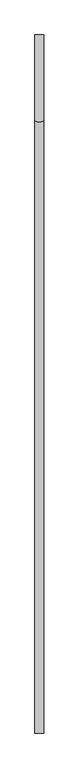
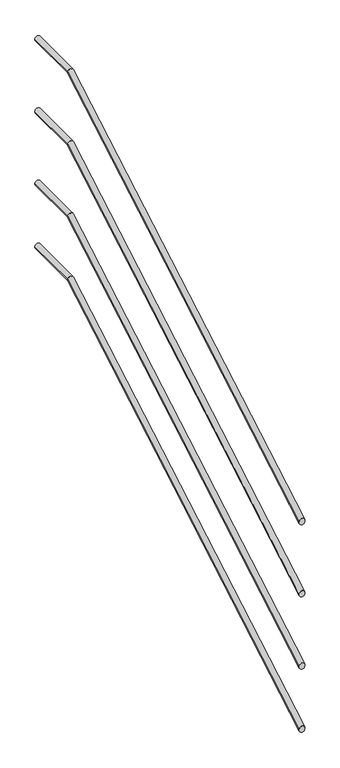
"""IFC4 building model written with IfcOpenShell, lengths in millimetres: railing geometry."""

import ifcopenshell
import ifcopenshell.guid

model = None  # the IFC model being written
_history = None  # IfcOwnerHistory: only IFC2X3 demands one
_inside = {}  # id of a spatial element -> (the spatial element, [elements in it])
_under = {}  # id of a project, library or spatial element -> (it, [spatial elements below it])
_declared = {}  # id of a project -> (the project, [libraries it declares])
_typed = {}  # id of a type object -> (the type object, [elements of that type])
_made_of = {}  # id of a material, layer set ... -> (it, [elements and type objects made of it])


def new_model(schema):
    """Start an empty IFC model of exactly this schema.

    Asked for "IFC4X3", IfcOpenShell would pick the latest addendum, in which some entities
    have other attributes; the version numbers below select the first issue.
    IFC2X3 requires an IfcOwnerHistory on every rooted entity: one is made here for all.
    """
    global model, _history
    if schema == "IFC4X3":
        model = ifcopenshell.file(schema_version=(4, 3, 0, 0))
    else:
        model = ifcopenshell.file(schema=schema)
    _inside.clear()
    _under.clear()
    _declared.clear()
    _typed.clear()
    _made_of.clear()
    _history = None
    if model.schema == "IFC2X3":
        org = make("IfcOrganization", Name="unknown")
        user = make(
            "IfcPersonAndOrganization",
            ThePerson=make("IfcPerson", FamilyName="unknown"),
            TheOrganization=org,
        )
        app = make(
            "IfcApplication",
            ApplicationDeveloper=org,
            Version="unknown",
            ApplicationFullName="unknown",
            ApplicationIdentifier="unknown",
        )
        _history = make(
            "IfcOwnerHistory",
            OwningUser=user,
            OwningApplication=app,
            ChangeAction="ADDED",
            CreationDate=0,
        )
    return model


def make(cls, **values):
    """One entity of the class cls with the attributes given. An attribute that is None is left unset."""
    return model.create_entity(
        cls, **{name: value for name, value in values.items() if value is not None}
    )


def rooted(cls, **values):
    """An entity with a GlobalId (a new one), such as an element, a storey or a relation."""
    return make(cls, GlobalId=ifcopenshell.guid.new(), OwnerHistory=_history, **values)


def si_unit(unit_type, name, prefix=None):
    """IfcSIUnit, for example si_unit("LENGTHUNIT", "METRE", prefix="MILLI")."""
    return make("IfcSIUnit", UnitType=unit_type, Prefix=prefix, Name=name)


def assignment(units):
    """IfcUnitAssignment: the units of a project."""
    return None if units is None else make("IfcUnitAssignment", Units=units)


def point(xyz):
    """IfcCartesianPoint."""
    return None if xyz is None else make("IfcCartesianPoint", Coordinates=xyz)


def direction(xyz):
    """IfcDirection."""
    return None if xyz is None else make("IfcDirection", DirectionRatios=xyz)


def frame(location, z_axis=None, x_axis=None):
    """IfcAxis2Placement3D, a coordinate frame: its origin and axes. An axis left out is left unset."""
    return make(
        "IfcAxis2Placement3D",
        Location=point(location),
        Axis=direction(z_axis),
        RefDirection=direction(x_axis),
    )


def origin():
    """The frame at (0, 0, 0) with its axes left unset."""
    return frame((0.0, 0.0, 0.0))


def place(relative_to, where):
    """IfcLocalPlacement: puts the frame where relative to a parent placement (None: the world)."""
    return make(
        "IfcLocalPlacement", PlacementRelTo=relative_to, RelativePlacement=where
    )


def context(
    kind, dimensions, precision=None, world=None, true_north=None, identifier=None
):
    """IfcGeometricRepresentationContext, for example the 3D "Model" context."""
    return make(
        "IfcGeometricRepresentationContext",
        ContextIdentifier=identifier,
        ContextType=kind,
        CoordinateSpaceDimension=dimensions,
        Precision=precision,
        WorldCoordinateSystem=world,
        TrueNorth=true_north,
    )


def project(units=None, contexts=None):
    """IfcProject with its units and contexts."""
    return rooted(
        "IfcProject",
        Name="project",
        RepresentationContexts=contexts,
        UnitsInContext=assignment(units),
    )


def spatial(cls, under=None, at=None, **own):
    """A site, building, storey or space (cls), placed at a placement, below another one or the project."""
    s = rooted(cls, ObjectPlacement=at, **own)
    if under is not None:
        _under.setdefault(under.id(), (under, []))[1].append(s)
    return s


def circle_curve(where, radius):
    """IfcCircle in the frame where."""
    return make("IfcCircle", Position=where, Radius=radius)


def ellipse_curve(where, semi_axis1, semi_axis2):
    """IfcEllipse in the frame where."""
    return make(
        "IfcEllipse", Position=where, SemiAxis1=semi_axis1, SemiAxis2=semi_axis2
    )


def shape(context_of_items, identifier, shape_type, items):
    """IfcShapeRepresentation: the items that make up one representation, for example the "Body"."""
    return make(
        "IfcShapeRepresentation",
        ContextOfItems=context_of_items,
        RepresentationIdentifier=identifier,
        RepresentationType=shape_type,
        Items=items,
    )


def source(mapping_origin, context_of_items, identifier, shape_type, items):
    """IfcRepresentationMap: a shape defined once, which mapped items show again and again."""
    return make(
        "IfcRepresentationMap",
        MappingOrigin=mapping_origin,
        MappedRepresentation=shape(context_of_items, identifier, shape_type, items),
    )


def transform(
    local_origin,
    x_axis=None,
    y_axis=None,
    z_axis=None,
    scale=None,
    scale2=None,
    scale3=None,
    uniform=True,
):
    """IfcCartesianTransformationOperator3D, or its non-uniform kind. x_axis, y_axis, z_axis: its Axis1, 2, 3."""
    if uniform:
        return make(
            "IfcCartesianTransformationOperator3D",
            Axis1=direction(x_axis),
            Axis2=direction(y_axis),
            LocalOrigin=point(local_origin),
            Scale=scale,
            Axis3=direction(z_axis),
        )
    return make(
        "IfcCartesianTransformationOperator3DnonUniform",
        Axis1=direction(x_axis),
        Axis2=direction(y_axis),
        LocalOrigin=point(local_origin),
        Scale=scale,
        Axis3=direction(z_axis),
        Scale2=scale2,
        Scale3=scale3,
    )


def mapped(mapping_source, mapping_target):
    """IfcMappedItem: shows the shape of a source again, moved by a transform."""
    return make(
        "IfcMappedItem", MappingSource=mapping_source, MappingTarget=mapping_target
    )


def made_of(thing, what):
    """Note that an element or type object is made of a material, layer set ...; save() writes the relation."""
    if what is not None:
        _made_of.setdefault(what.id(), (what, []))[1].append(thing)
    return thing


def element(
    cls,
    number,
    at=None,
    inside=None,
    cuts=None,
    type_object=None,
    material=None,
    context=None,
    identifier="Body",
    shape_type=None,
    held_by="IfcProductDefinitionShape",
    body=None,
    shapes=None,
    **own,
):
    """One element of the class cls, such as IfcWall. Its Tag is "e" and its number.

    at: its placement. inside: the storey or other place that contains it. cuts: it is an
    opening in that element (IfcRelVoidsElement). A single representation is given by context,
    identifier, shape_type and body (its items); several are given by shapes. held_by: the class
    of the entity that holds the representations. save() writes the other relations.
    """
    e = rooted(cls, Tag="e%d" % number, ObjectPlacement=at, **own)
    if body is not None:
        shapes = [shape(context, identifier, shape_type, body)]
    if shapes is not None:
        e.Representation = make(held_by, Representations=shapes)
    if inside is not None:
        _inside.setdefault(inside.id(), (inside, []))[1].append(e)
    if cuts is not None:
        rooted(
            "IfcRelVoidsElement", RelatingBuildingElement=cuts, RelatedOpeningElement=e
        )
    if type_object is not None:
        _typed.setdefault(type_object.id(), (type_object, []))[1].append(e)
    return made_of(e, material)


def aggregate(whole, parts):
    """IfcRelAggregates: a whole, such as a stair, and the parts it consists of."""
    return rooted("IfcRelAggregates", RelatingObject=whole, RelatedObjects=parts)


def save(model, path):
    """Write the relations noted so far, then the file.

    IfcRelAggregates (storeys below a building ...), IfcRelContainedInSpatialStructure (elements
    in a storey), IfcRelDefinesByType, IfcRelAssociatesMaterial and IfcRelDeclares: one each for
    every whole, place, type object, material and project.
    """
    for whole, parts in _under.values():
        aggregate(whole, parts)
    for where, things in _inside.values():
        rooted(
            "IfcRelContainedInSpatialStructure",
            RelatedElements=things,
            RelatingStructure=where,
        )
    for kind, things in _typed.values():
        rooted("IfcRelDefinesByType", RelatedObjects=things, RelatingType=kind)
    for what, things in _made_of.values():
        rooted("IfcRelAssociatesMaterial", RelatedObjects=things, RelatingMaterial=what)
    for by, libraries in _declared.values():
        rooted("IfcRelDeclares", RelatingContext=by, RelatedDefinitions=libraries)
    model.write(path)


def plane_surface(at):
    """IfcPlane: the flat surface through the origin of the frame at, square to its z axis."""
    return make("IfcPlane", Position=at)


def cylinder_surface(at, radius):
    """IfcCylindricalSurface: all points at the distance radius from the z axis of the frame at."""
    return make("IfcCylindricalSurface", Position=at, Radius=radius)


def advanced_brep(points, edges, surfaces, faces):
    """IfcAdvancedBrep: a solid bounded by faces that lie on surfaces and meet in shared edges.

    An edge is (start, end): straight between two places in points (the first is 0);
    or (start, end, curve); or (start, end, curve, False) where it runs against its curve.
    A face is (place in surfaces, loops), or (place, loops, False) where it looks against
    its surface's normal. A loop lists edges by number (the first is 1), with a minus sign
    where the edge is run from its end to its start. The first loop is the outer one.
    """
    corners = [point(p) for p in points]
    vertices = [make("IfcVertexPoint", VertexGeometry=c) for c in corners]
    made = []
    for start, end, *more in edges:
        made.append(
            make(
                "IfcEdgeCurve",
                EdgeStart=vertices[start],
                EdgeEnd=vertices[end],
                EdgeGeometry=more[0] if more else make("IfcPolyline", Points=[corners[start], corners[end]]),
                SameSense=more[1] if len(more) > 1 else True,
            )
        )
    hull = []
    for where, loops, *sense in faces:
        bounds = []
        for j, loop in enumerate(loops):
            ring = [make("IfcOrientedEdge", EdgeElement=made[abs(k) - 1], Orientation=k > 0) for k in loop]
            bounds.append(
                make(
                    "IfcFaceOuterBound" if j == 0 else "IfcFaceBound",
                    Bound=make("IfcEdgeLoop", EdgeList=ring),
                    Orientation=True,
                )
            )
        hull.append(make("IfcAdvancedFace", Bounds=bounds, FaceSurface=surfaces[where], SameSense=sense[0] if sense else True))
    return make("IfcAdvancedBrep", Outer=make("IfcClosedShell", CfsFaces=hull))


def railing_e49ed630(model_context):
    return source(origin(), model_context, "Body", "AdvancedBrep", [
        advanced_brep(
        [(-1890.4, 13399.5208589, 1336.7361432), (-1860.4, 13399.5208589, 1336.7361432), (-1890.4, 15503.5584173, 2557.9030398), (-1860.4, 15503.5584173, 2557.9030398), (-1890.4, 15799.5208589, 2557.9030398), (-1860.4, 15799.5208589, 2557.9030398)],
        [
            (0, 1, ellipse_curve(frame((-1875.4, 13399.5208589, 1336.7361432), z_axis=(0.0, -1.0, 0.0), x_axis=(0.0, 0.0, -1.0)), 17.3433672, 15.0)),
            (1, 0, ellipse_curve(frame((-1875.4, 13399.5208589, 1336.7361432), z_axis=(0.0, -1.0, 0.0), x_axis=(0.0, 0.0, -1.0)), 17.3433672, 15.0)),
            (0, 2),
            (2, 3, ellipse_curve(frame((-1875.4, 15503.5584173, 2557.9030398), z_axis=(0.0, -0.9656303515230846, -0.25991926480621624), x_axis=(0.0, 0.2599192648062163, -0.9656303515230846)), 15.5338945, 15.0)),
            (3, 1),
            (3, 2, ellipse_curve(frame((-1875.4, 15503.5584173, 2557.9030398), z_axis=(0.0, -0.9656303515230846, -0.25991926480621624), x_axis=(0.0, 0.2599192648062163, -0.9656303515230846)), 15.5338945, 15.0)),
            (4, 5, circle_curve(frame((-1875.4, 15799.5208589, 2557.9030398), z_axis=(0.0, 1.0, 0.0), x_axis=(1.0, 0.0, 0.0)), 15.0)),
            (5, 4, circle_curve(frame((-1875.4, 15799.5208589, 2557.9030398), z_axis=(0.0, 1.0, 0.0), x_axis=(1.0, 0.0, 0.0)), 15.0)),
            (2, 4),
            (5, 3),
        ],
        [
            plane_surface(frame((-1875.4, 13399.5208589, 1354.0795104), z_axis=(0.0, -1.0, 0.0), x_axis=(0.0, 0.0, 1.0))),
            cylinder_surface(frame((-1875.4, 13407.0504368, 1341.1062512), z_axis=(0.0, -0.864883951565192, -0.5019718620848966), x_axis=(1.0, 0.0, 0.0)), 15.0),
            plane_surface(frame((-1875.4, 15799.5208589, 2572.9030398), z_axis=(0.0, 1.0, 0.0), x_axis=(0.0, 0.0, 1.0))),
            cylinder_surface(frame((-1875.4, 15499.5208589, 2557.9030398), z_axis=(0.0, -1.0, 0.0), x_axis=(1.0, 0.0, 0.0)), 15.0),
        ],
        [
            (0, [[1, 2]]),
            (1, [[-1, 3, 4, 5]]),
            (1, [[-2, -5, 6, -3]]),
            (2, [[7, 8]]),
            (3, [[-4, 9, -8, 10]]),
            (3, [[-6, -10, -7, -9]]),
        ],
    ),
        advanced_brep(
        [(-1890.4, 13399.5208589, 536.7361432), (-1860.4, 13399.5208589, 536.7361432), (-1890.4, 15503.5584173, 1757.9030398), (-1860.4, 15503.5584173, 1757.9030398), (-1890.4, 15799.5208589, 1757.9030398), (-1860.4, 15799.5208589, 1757.9030398)],
        [
            (0, 1, ellipse_curve(frame((-1875.4, 13399.5208589, 536.7361432), z_axis=(0.0, -1.0, 0.0), x_axis=(0.0, 0.0, -1.0)), 17.3433672, 15.0)),
            (1, 0, ellipse_curve(frame((-1875.4, 13399.5208589, 536.7361432), z_axis=(0.0, -1.0, 0.0), x_axis=(0.0, 0.0, -1.0)), 17.3433672, 15.0)),
            (0, 2),
            (2, 3, ellipse_curve(frame((-1875.4, 15503.5584173, 1757.9030398), z_axis=(0.0, -0.9656303515230846, -0.25991926480621624), x_axis=(0.0, 0.2599192648062163, -0.9656303515230846)), 15.5338945, 15.0)),
            (3, 1),
            (3, 2, ellipse_curve(frame((-1875.4, 15503.5584173, 1757.9030398), z_axis=(0.0, -0.9656303515230846, -0.25991926480621624), x_axis=(0.0, 0.2599192648062163, -0.9656303515230846)), 15.5338945, 15.0)),
            (4, 5, circle_curve(frame((-1875.4, 15799.5208589, 1757.9030398), z_axis=(0.0, 1.0, 0.0), x_axis=(1.0, 0.0, 0.0)), 15.0)),
            (5, 4, circle_curve(frame((-1875.4, 15799.5208589, 1757.9030398), z_axis=(0.0, 1.0, 0.0), x_axis=(1.0, 0.0, 0.0)), 15.0)),
            (2, 4),
            (5, 3),
        ],
        [
            plane_surface(frame((-1875.4, 13399.5208589, 554.0795104), z_axis=(0.0, -1.0, 0.0), x_axis=(0.0, 0.0, 1.0))),
            cylinder_surface(frame((-1875.4, 13407.0504368, 541.1062512), z_axis=(0.0, -0.864883951565192, -0.5019718620848966), x_axis=(1.0, 0.0, 0.0)), 15.0),
            plane_surface(frame((-1875.4, 15799.5208589, 1772.9030398), z_axis=(0.0, 1.0, 0.0), x_axis=(0.0, 0.0, 1.0))),
            cylinder_surface(frame((-1875.4, 15499.5208589, 1757.9030398), z_axis=(0.0, -1.0, 0.0), x_axis=(1.0, 0.0, 0.0)), 15.0),
        ],
        [
            (0, [[1, 2]]),
            (1, [[-1, 3, 4, 5]]),
            (1, [[-2, -5, 6, -3]]),
            (2, [[7, 8]]),
            (3, [[-4, 9, -8, 10]]),
            (3, [[-6, -10, -7, -9]]),
        ],
    ),
        advanced_brep(
        [(-1890.4, 13399.5208589, 936.7361432), (-1860.4, 13399.5208589, 936.7361432), (-1890.4, 15503.5584173, 2157.9030398), (-1860.4, 15503.5584173, 2157.9030398), (-1890.4, 15799.5208589, 2157.9030398), (-1860.4, 15799.5208589, 2157.9030398)],
        [
            (0, 1, ellipse_curve(frame((-1875.4, 13399.5208589, 936.7361432), z_axis=(0.0, -1.0, 0.0), x_axis=(0.0, 0.0, -1.0)), 17.3433672, 15.0)),
            (1, 0, ellipse_curve(frame((-1875.4, 13399.5208589, 936.7361432), z_axis=(0.0, -1.0, 0.0), x_axis=(0.0, 0.0, -1.0)), 17.3433672, 15.0)),
            (0, 2),
            (2, 3, ellipse_curve(frame((-1875.4, 15503.5584173, 2157.9030398), z_axis=(0.0, -0.9656303515230846, -0.25991926480621624), x_axis=(0.0, 0.2599192648062163, -0.9656303515230846)), 15.5338945, 15.0)),
            (3, 1),
            (3, 2, ellipse_curve(frame((-1875.4, 15503.5584173, 2157.9030398), z_axis=(0.0, -0.9656303515230846, -0.25991926480621624), x_axis=(0.0, 0.2599192648062163, -0.9656303515230846)), 15.5338945, 15.0)),
            (4, 5, circle_curve(frame((-1875.4, 15799.5208589, 2157.9030398), z_axis=(0.0, 1.0, 0.0), x_axis=(1.0, 0.0, 0.0)), 15.0)),
            (5, 4, circle_curve(frame((-1875.4, 15799.5208589, 2157.9030398), z_axis=(0.0, 1.0, 0.0), x_axis=(1.0, 0.0, 0.0)), 15.0)),
            (2, 4),
            (5, 3),
        ],
        [
            plane_surface(frame((-1875.4, 13399.5208589, 954.0795104), z_axis=(0.0, -1.0, 0.0), x_axis=(0.0, 0.0, 1.0))),
            cylinder_surface(frame((-1875.4, 13407.0504368, 941.1062512), z_axis=(0.0, -0.864883951565192, -0.5019718620848966), x_axis=(1.0, 0.0, 0.0)), 15.0),
            plane_surface(frame((-1875.4, 15799.5208589, 2172.9030398), z_axis=(0.0, 1.0, 0.0), x_axis=(0.0, 0.0, 1.0))),
            cylinder_surface(frame((-1875.4, 15499.5208589, 2157.9030398), z_axis=(0.0, -1.0, 0.0), x_axis=(1.0, 0.0, 0.0)), 15.0),
        ],
        [
            (0, [[1, 2]]),
            (1, [[-1, 3, 4, 5]]),
            (1, [[-2, -5, 6, -3]]),
            (2, [[7, 8]]),
            (3, [[-4, 9, -8, 10]]),
            (3, [[-6, -10, -7, -9]]),
        ],
    ),
        advanced_brep(
        [(-1890.4, 13399.5208589, 186.7361432), (-1860.4, 13399.5208589, 186.7361432), (-1890.4, 15503.5584173, 1407.9030398), (-1860.4, 15503.5584173, 1407.9030398), (-1890.4, 15799.5208589, 1407.9030398), (-1860.4, 15799.5208589, 1407.9030398)],
        [
            (0, 1, ellipse_curve(frame((-1875.4, 13399.5208589, 186.7361432), z_axis=(0.0, -1.0, 0.0), x_axis=(0.0, 0.0, -1.0)), 17.3433672, 15.0)),
            (1, 0, ellipse_curve(frame((-1875.4, 13399.5208589, 186.7361432), z_axis=(0.0, -1.0, 0.0), x_axis=(0.0, 0.0, -1.0)), 17.3433672, 15.0)),
            (0, 2),
            (2, 3, ellipse_curve(frame((-1875.4, 15503.5584173, 1407.9030398), z_axis=(0.0, -0.9656303515230846, -0.25991926480621624), x_axis=(0.0, 0.2599192648062163, -0.9656303515230846)), 15.5338945, 15.0)),
            (3, 1),
            (3, 2, ellipse_curve(frame((-1875.4, 15503.5584173, 1407.9030398), z_axis=(0.0, -0.9656303515230846, -0.25991926480621624), x_axis=(0.0, 0.2599192648062163, -0.9656303515230846)), 15.5338945, 15.0)),
            (4, 5, circle_curve(frame((-1875.4, 15799.5208589, 1407.9030398), z_axis=(0.0, 1.0, 0.0), x_axis=(1.0, 0.0, 0.0)), 15.0)),
            (5, 4, circle_curve(frame((-1875.4, 15799.5208589, 1407.9030398), z_axis=(0.0, 1.0, 0.0), x_axis=(1.0, 0.0, 0.0)), 15.0)),
            (2, 4),
            (5, 3),
        ],
        [
            plane_surface(frame((-1875.4, 13399.5208589, 204.0795104), z_axis=(0.0, -1.0, 0.0), x_axis=(0.0, 0.0, 1.0))),
            cylinder_surface(frame((-1875.4, 13407.0504368, 191.1062512), z_axis=(0.0, -0.864883951565192, -0.5019718620848966), x_axis=(1.0, 0.0, 0.0)), 15.0),
            plane_surface(frame((-1875.4, 15799.5208589, 1422.9030398), z_axis=(0.0, 1.0, 0.0), x_axis=(0.0, 0.0, 1.0))),
            cylinder_surface(frame((-1875.4, 15499.5208589, 1407.9030398), z_axis=(0.0, -1.0, 0.0), x_axis=(1.0, 0.0, 0.0)), 15.0),
        ],
        [
            (0, [[1, 2]]),
            (1, [[-1, 3, 4, 5]]),
            (1, [[-2, -5, 6, -3]]),
            (2, [[7, 8]]),
            (3, [[-4, 9, -8, 10]]),
            (3, [[-6, -10, -7, -9]]),
        ],
    ),
    ])


if __name__ == "__main__":
    model = new_model("IFC4")
    model_context = context("Model", 3, world=origin())
    ifc_project = project(units=[si_unit("LENGTHUNIT", "METRE", prefix="MILLI")], contexts=[model_context])
    site = spatial("IfcSite", under=ifc_project)
    building = spatial("IfcBuilding", under=site)
    placement = place(None, origin())
    railing_shape = railing_e49ed630(model_context)
    element("IfcRailing", 1, at=placement, inside=building, context=model_context, shape_type="MappedRepresentation", body=[
        mapped(railing_shape, transform((0.0, 0.0, 0.0), x_axis=(1.0, 0.0, 0.0), y_axis=(0.0, 1.0, 0.0), z_axis=(0.0, 0.0, 1.0))),
    ])
    save(model, "model.ifc")
